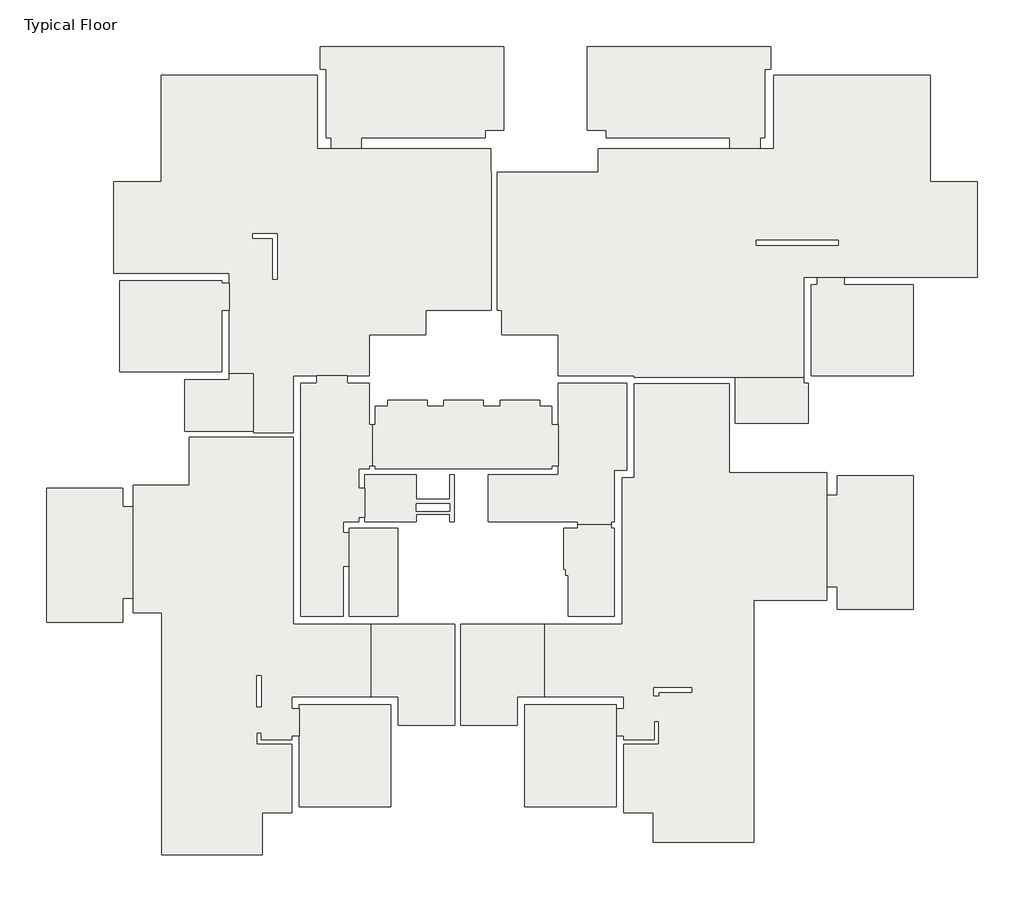
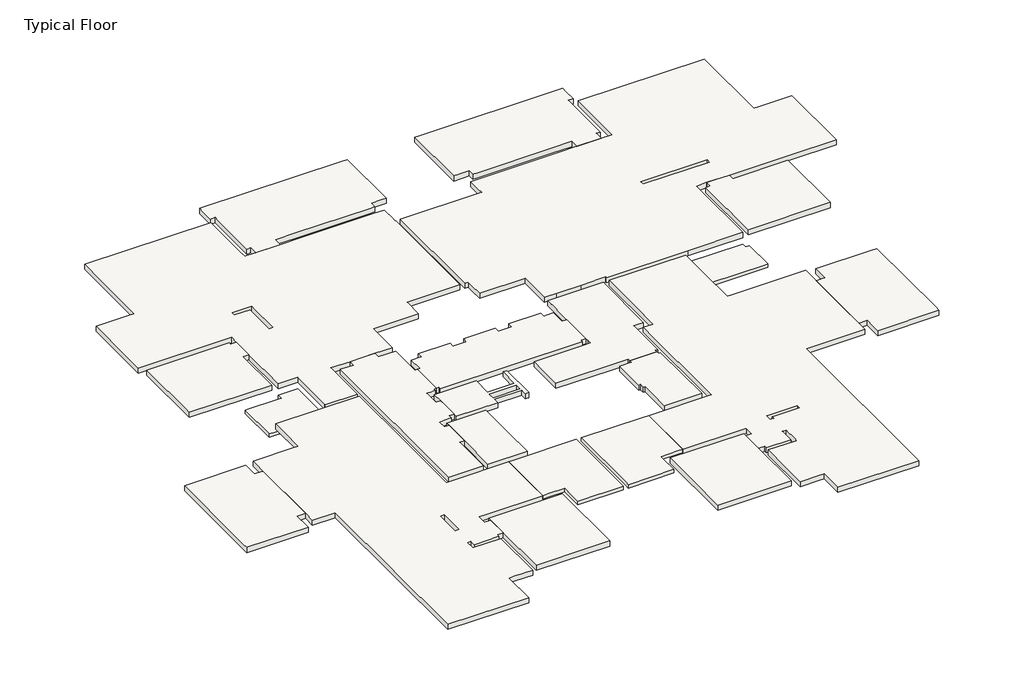
# One storey: 22 slabs.
"""IFC4 building model written with IfcOpenShell, lengths in millimetres."""

import ifcopenshell
import ifcopenshell.guid

model = None  # the IFC model being written
_history = None  # IfcOwnerHistory: only IFC2X3 demands one
_inside = {}  # id of a spatial element -> (the spatial element, [elements in it])
_under = {}  # id of a project, library or spatial element -> (it, [spatial elements below it])
_declared = {}  # id of a project -> (the project, [libraries it declares])
_typed = {}  # id of a type object -> (the type object, [elements of that type])
_made_of = {}  # id of a material, layer set ... -> (it, [elements and type objects made of it])


def new_model(schema):
    """Start an empty IFC model of exactly this schema.

    Asked for "IFC4X3", IfcOpenShell would pick the latest addendum, in which some entities
    have other attributes; the version numbers below select the first issue.
    IFC2X3 requires an IfcOwnerHistory on every rooted entity: one is made here for all.
    """
    global model, _history
    if schema == "IFC4X3":
        model = ifcopenshell.file(schema_version=(4, 3, 0, 0))
    else:
        model = ifcopenshell.file(schema=schema)
    _inside.clear()
    _under.clear()
    _declared.clear()
    _typed.clear()
    _made_of.clear()
    _history = None
    if model.schema == "IFC2X3":
        org = make("IfcOrganization", Name="unknown")
        user = make(
            "IfcPersonAndOrganization",
            ThePerson=make("IfcPerson", FamilyName="unknown"),
            TheOrganization=org,
        )
        app = make(
            "IfcApplication",
            ApplicationDeveloper=org,
            Version="unknown",
            ApplicationFullName="unknown",
            ApplicationIdentifier="unknown",
        )
        _history = make(
            "IfcOwnerHistory",
            OwningUser=user,
            OwningApplication=app,
            ChangeAction="ADDED",
            CreationDate=0,
        )
    return model


def make(cls, **values):
    """One entity of the class cls with the attributes given. An attribute that is None is left unset."""
    return model.create_entity(
        cls, **{name: value for name, value in values.items() if value is not None}
    )


def rooted(cls, **values):
    """An entity with a GlobalId (a new one), such as an element, a storey or a relation."""
    return make(cls, GlobalId=ifcopenshell.guid.new(), OwnerHistory=_history, **values)


def si_unit(unit_type, name, prefix=None):
    """IfcSIUnit, for example si_unit("LENGTHUNIT", "METRE", prefix="MILLI")."""
    return make("IfcSIUnit", UnitType=unit_type, Prefix=prefix, Name=name)


def assignment(units):
    """IfcUnitAssignment: the units of a project."""
    return None if units is None else make("IfcUnitAssignment", Units=units)


def point(xyz):
    """IfcCartesianPoint."""
    return None if xyz is None else make("IfcCartesianPoint", Coordinates=xyz)


def direction(xyz):
    """IfcDirection."""
    return None if xyz is None else make("IfcDirection", DirectionRatios=xyz)


def frame(location, z_axis=None, x_axis=None):
    """IfcAxis2Placement3D, a coordinate frame: its origin and axes. An axis left out is left unset."""
    return make(
        "IfcAxis2Placement3D",
        Location=point(location),
        Axis=direction(z_axis),
        RefDirection=direction(x_axis),
    )


def origin():
    """The frame at (0, 0, 0) with its axes left unset."""
    return frame((0.0, 0.0, 0.0))


def place(relative_to, where):
    """IfcLocalPlacement: puts the frame where relative to a parent placement (None: the world)."""
    return make(
        "IfcLocalPlacement", PlacementRelTo=relative_to, RelativePlacement=where
    )


def context(
    kind, dimensions, precision=None, world=None, true_north=None, identifier=None
):
    """IfcGeometricRepresentationContext, for example the 3D "Model" context."""
    return make(
        "IfcGeometricRepresentationContext",
        ContextIdentifier=identifier,
        ContextType=kind,
        CoordinateSpaceDimension=dimensions,
        Precision=precision,
        WorldCoordinateSystem=world,
        TrueNorth=true_north,
    )


def project(units=None, contexts=None):
    """IfcProject with its units and contexts."""
    return rooted(
        "IfcProject",
        Name="project",
        RepresentationContexts=contexts,
        UnitsInContext=assignment(units),
    )


def spatial(cls, under=None, at=None, **own):
    """A site, building, storey or space (cls), placed at a placement, below another one or the project."""
    s = rooted(cls, ObjectPlacement=at, **own)
    if under is not None:
        _under.setdefault(under.id(), (under, []))[1].append(s)
    return s


def polyline(points):
    """IfcPolyline through the points."""
    return make("IfcPolyline", Points=[point(p) for p in points])


def outline(outer, holes=None, kind="AREA"):
    """IfcArbitraryClosedProfileDef: a profile drawn as a closed curve; with holes, ...WithVoids."""
    if holes is None:
        return make("IfcArbitraryClosedProfileDef", ProfileType=kind, OuterCurve=outer)
    return make(
        "IfcArbitraryProfileDefWithVoids",
        ProfileType=kind,
        OuterCurve=outer,
        InnerCurves=holes,
    )


def extrude(swept, where, along, depth):
    """IfcExtrudedAreaSolid: the profile swept, set in the frame where, extruded along a direction by depth."""
    return make(
        "IfcExtrudedAreaSolid",
        SweptArea=swept,
        Position=where,
        ExtrudedDirection=direction(along),
        Depth=depth,
    )


def faces_of(points, faces, orient=None, outer=None):
    """IfcFace entities. A face is a list of loops; a loop is a list of indices into points, from 0.

    orient and outer hold one flag for each loop. By default every Orientation is true, the
    first loop of a face is its IfcFaceOuterBound and the others are IfcFaceBound.
    """
    made = []
    for i, loops in enumerate(faces):
        bounds = []
        for j, loop in enumerate(loops):
            is_outer = j == 0 if outer is None else outer[i][j]
            bounds.append(
                make(
                    "IfcFaceOuterBound" if is_outer else "IfcFaceBound",
                    Bound=make("IfcPolyLoop", Polygon=[points[k] for k in loop]),
                    Orientation=True if orient is None else orient[i][j],
                )
            )
        made.append(make("IfcFace", Bounds=bounds))
    return made


def faceted_brep(points, faces, orient=None, outer=None, voids=None):
    """IfcFacetedBrep: a solid bounded by flat faces; with voids (closed shells), ...WithVoids."""
    shared = [point(p) for p in points]
    hull = make("IfcClosedShell", CfsFaces=faces_of(shared, faces, orient, outer))
    if voids is None:
        return make("IfcFacetedBrep", Outer=hull)
    return make(
        "IfcFacetedBrepWithVoids",
        Outer=hull,
        Voids=[
            make(cls, CfsFaces=faces_of(shared, fs, o, b)) for cls, fs, o, b in voids
        ],
    )


def shape(context_of_items, identifier, shape_type, items):
    """IfcShapeRepresentation: the items that make up one representation, for example the "Body"."""
    return make(
        "IfcShapeRepresentation",
        ContextOfItems=context_of_items,
        RepresentationIdentifier=identifier,
        RepresentationType=shape_type,
        Items=items,
    )


def made_of(thing, what):
    """Note that an element or type object is made of a material, layer set ...; save() writes the relation."""
    if what is not None:
        _made_of.setdefault(what.id(), (what, []))[1].append(thing)
    return thing


def element(
    cls,
    number,
    at=None,
    inside=None,
    cuts=None,
    type_object=None,
    material=None,
    context=None,
    identifier="Body",
    shape_type=None,
    held_by="IfcProductDefinitionShape",
    body=None,
    shapes=None,
    **own,
):
    """One element of the class cls, such as IfcWall. Its Tag is "e" and its number.

    at: its placement. inside: the storey or other place that contains it. cuts: it is an
    opening in that element (IfcRelVoidsElement). A single representation is given by context,
    identifier, shape_type and body (its items); several are given by shapes. held_by: the class
    of the entity that holds the representations. save() writes the other relations.
    """
    e = rooted(cls, Tag="e%d" % number, ObjectPlacement=at, **own)
    if body is not None:
        shapes = [shape(context, identifier, shape_type, body)]
    if shapes is not None:
        e.Representation = make(held_by, Representations=shapes)
    if inside is not None:
        _inside.setdefault(inside.id(), (inside, []))[1].append(e)
    if cuts is not None:
        rooted(
            "IfcRelVoidsElement", RelatingBuildingElement=cuts, RelatedOpeningElement=e
        )
    if type_object is not None:
        _typed.setdefault(type_object.id(), (type_object, []))[1].append(e)
    return made_of(e, material)


def aggregate(whole, parts):
    """IfcRelAggregates: a whole, such as a stair, and the parts it consists of."""
    return rooted("IfcRelAggregates", RelatingObject=whole, RelatedObjects=parts)


def save(model, path):
    """Write the relations noted so far, then the file.

    IfcRelAggregates (storeys below a building ...), IfcRelContainedInSpatialStructure (elements
    in a storey), IfcRelDefinesByType, IfcRelAssociatesMaterial and IfcRelDeclares: one each for
    every whole, place, type object, material and project.
    """
    for whole, parts in _under.values():
        aggregate(whole, parts)
    for where, things in _inside.values():
        rooted(
            "IfcRelContainedInSpatialStructure",
            RelatedElements=things,
            RelatingStructure=where,
        )
    for kind, things in _typed.values():
        rooted("IfcRelDefinesByType", RelatedObjects=things, RelatingType=kind)
    for what, things in _made_of.values():
        rooted("IfcRelAssociatesMaterial", RelatedObjects=things, RelatingMaterial=what)
    for by, libraries in _declared.values():
        rooted("IfcRelDeclares", RelatingContext=by, RelatedDefinitions=libraries)
    model.write(path)


model = new_model("IFC4")

# Units and contexts
model_context = context("Model", 3, world=origin())
ifc_project = project(units=[si_unit("LENGTHUNIT", "METRE", prefix="MILLI")], contexts=[model_context])

# Site, building, storey
site = spatial("IfcSite", under=ifc_project)
building = spatial("IfcBuilding", under=site)
storey = spatial("IfcBuildingStorey", under=building, Name="Typical Floor", Elevation=3100.0)

# Slabs
placement = place(None, origin())
element("IfcSlab", 1, ObjectType="15", at=placement, inside=storey, context=model_context, shape_type="Brep", body=[
    faceted_brep([(26027.850174, -8804.7310591, 2300.0), (26027.850174, -9003.4933914, 2300.0), (26177.850174, -9003.4933914, 2300.0), (26177.850174, -10305.7627314, 2300.0), (23780.6220263, -10305.7627314, 2300.0), (23780.6220263, -8804.7310591, 2300.0), (26027.850174, -9003.4933914, 2450.0), (26027.850174, -8954.7310591, 2450.0), (26027.850174, -8804.7310591, 2450.0), (23780.6220263, -8804.7310591, 2450.0), (23780.6220263, -8954.7310591, 2450.0), (23780.6220263, -10305.7627314, 2450.0), (26027.850174, -10305.7627314, 2450.0), (26177.850174, -10305.7627314, 2450.0), (26177.850174, -9003.4933914, 2450.0)], [[[0, 1, 2, 3, 4, 5]], [[6, 7, 8, 9, 10, 11, 12, 13, 14]], [[1, 0, 8, 7, 6]], [[2, 1, 6, 14]], [[3, 2, 14, 13]], [[4, 3, 13, 12, 11]], [[5, 4, 11, 10, 9]], [[0, 5, 9, 8]]]),
])
element("IfcSlab", 2, ObjectType="15", at=placement, inside=storey, context=model_context, shape_type="Brep", body=[
    faceted_brep([(5696.9503171, -10574.5447275, 2300.0), (5696.9503171, -8875.9821525, 2300.0), (6907.9504595, -8875.9821525, 2300.0), (7157.9504595, -8875.9821525, 2300.0), (7157.9504595, -8673.5161743, 2300.0), (7954.0579731, -8673.5161743, 2300.0), (7954.0579731, -10574.5447275, 2300.0), (5696.9503171, -8875.9821525, 2450.0), (5696.9503171, -10574.5447275, 2450.0), (5846.9503171, -10574.5447275, 2450.0), (7804.0579731, -10574.5447275, 2450.0), (7954.0579731, -10574.5447275, 2450.0), (7954.0579731, -8873.5161743, 2450.0), (7954.0579731, -8673.5161743, 2450.0), (7157.9504595, -8673.5161743, 2450.0), (7157.9504595, -8873.5161743, 2450.0), (7157.9504595, -8875.9821525, 2450.0), (6907.9504595, -8875.9821525, 2450.0), (5846.9503171, -8875.9821525, 2450.0)], [[[0, 1, 2, 3, 4, 5, 6]], [[7, 8, 9, 10, 11, 12, 13, 14, 15, 16, 17, 18]], [[1, 0, 8, 7]], [[1, 7, 18, 17, 16, 3, 2]], [[4, 3, 16, 15, 14]], [[5, 4, 14, 13]], [[6, 5, 13, 12, 11]], [[0, 6, 11, 10, 9, 8]]]),
])
element("IfcSlab", 3, ObjectType="15", at=placement, inside=storey, context=model_context, shape_type="Brep", body=[
    faceted_brep([(11800.0437745, -19301.9218456, 2800.0), (11800.0437745, -16906.0156488, 2800.0), (12000.0437745, -16906.0156488, 2800.0), (14556.9532328, -16906.0156488, 2800.0), (14556.9532328, -20074.3060494, 2800.0), (14556.9532328, -20224.3060494, 2800.0), (12702.1320718, -20224.3060494, 2800.0), (12702.1320718, -20074.3060494, 2800.0), (12702.1320718, -19551.9218456, 2800.0), (12702.1320718, -19301.9218456, 2800.0), (12000.0437745, -19301.9218456, 2800.0), (11800.0437745, -16906.0156488, 2950.0), (11800.0437745, -19301.9218456, 2950.0), (12000.0437745, -19301.9218456, 2950.0), (12702.1320718, -19301.9218456, 2950.0), (12702.1320718, -19551.9218456, 2950.0), (12702.1320718, -20074.3060494, 2950.0), (12702.1320718, -20224.3060494, 2950.0), (14556.9532328, -20224.3060494, 2950.0), (14556.9532328, -20074.3060494, 2950.0), (14556.9532328, -16906.0156488, 2950.0), (12000.0437745, -16906.0156488, 2950.0)], [[[0, 1, 2, 3, 4, 5, 6, 7, 8, 9, 10]], [[11, 12, 13, 14, 15, 16, 17, 18, 19, 20, 21]], [[1, 0, 12, 11]], [[3, 2, 1, 11, 21, 20]], [[5, 4, 3, 20, 19, 18]], [[6, 5, 18, 17]], [[6, 17, 16, 15, 14, 9, 8, 7]], [[0, 10, 9, 14, 13, 12]]]),
])
element("IfcSlab", 4, ObjectType="15", at=placement, inside=storey, context=model_context, shape_type="Brep", body=[
    faceted_brep([(17508.6310988, -16906.0156488, 2800.0), (17508.6310988, -19301.9218456, 2800.0), (17308.6310988, -19301.9218456, 2800.0), (16611.7743938, -19301.9218456, 2800.0), (16611.7743938, -19551.9218456, 2800.0), (16611.7743938, -20074.3060494, 2800.0), (16611.7743938, -20224.3060494, 2800.0), (14756.9532328, -20224.3060494, 2800.0), (14756.9532328, -20074.3060494, 2800.0), (14756.9532328, -16906.0156488, 2800.0), (17308.6310988, -16906.0156488, 2800.0), (17508.6310988, -19301.9218456, 2950.0), (17508.6310988, -16906.0156488, 2950.0), (17308.6310988, -16906.0156488, 2950.0), (14756.9532328, -16906.0156488, 2950.0), (14756.9532328, -20074.3060494, 2950.0), (14756.9532328, -20224.3060494, 2950.0), (16611.7743938, -20224.3060494, 2950.0), (16611.7743938, -20074.3060494, 2950.0), (16611.7743938, -19551.9218456, 2950.0), (16611.7743938, -19301.9218456, 2950.0), (17308.6310988, -19301.9218456, 2950.0)], [[[0, 1, 2, 3, 4, 5, 6, 7, 8, 9, 10]], [[11, 12, 13, 14, 15, 16, 17, 18, 19, 20, 21]], [[1, 0, 12, 11]], [[3, 2, 1, 11, 21, 20]], [[3, 20, 19, 18, 17, 6, 5, 4]], [[7, 6, 17, 16]], [[9, 8, 7, 16, 15, 14]], [[0, 10, 9, 14, 13, 12]]]),
])
element("IfcSlab", 5, ObjectType="22", at=placement, inside=storey, context=model_context, shape_type="Brep", body=[
    faceted_brep([(7954.0579731, -8673.5161743, 2730.0), (7157.9504595, -8673.5161743, 2730.0), (7157.9504595, -6598.7689899, 2730.0), (7157.9504595, -5710.0703278, 2730.0), (7157.9504595, -5376.3894647, 2730.0), (6907.9504595, -5376.3894647, 2730.0), (3357.3073849, -5376.3894647, 2730.0), (3357.3073849, -2383.1380866, 2730.0), (4715.8368705, -2383.1380866, 2730.0), (4915.8368705, -2383.1380866, 2730.0), (4915.8368705, 1116.275118, 2730.0), (10045.0259753, 1116.275118, 2730.0), (10045.0259753, -935.8943434, 2730.0), (10045.0259753, -1285.8943434, 2730.0), (10497.5809154, -1285.8943434, 2730.0), (11496.1544072, -1285.8943434, 2730.0), (12338.469313, -1285.8943434, 2730.0), (15339.3043472, -1285.8943434, 2730.0), (15752.9774125, -1285.8943434, 2730.0), (15752.9774125, -1861.9790741, 2730.0), (15752.9774125, -2061.9790741, 2730.0), (15755.4299651, -2061.9790741, 2730.0), (15755.4299651, -6603.7071845, 2730.0), (13854.4950523, -6603.7071845, 2730.0), (13604.5871332, -6603.7071845, 2730.0), (13604.5871332, -7403.6947082, 2730.0), (12004.8805309, -7403.6947082, 2730.0), (11754.8805309, -7403.6947082, 2730.0), (11754.8805309, -8753.4091082, 2730.0), (11034.9623053, -8753.4091082, 2730.0), (10036.3888134, -8753.4091082, 2730.0), (9252.6267863, -8753.4091082, 2730.0), (9252.6267863, -9003.4091082, 2730.0), (9252.6267863, -10624.4557657, 2730.0), (7954.0579731, -10624.4557657, 2730.0), (7954.0579731, -10574.5447275, 2730.0), (7932.894282, -4076.5861029, 2730.0), (7932.894282, -4226.5861029, 2730.0), (8577.767247, -4226.5861029, 2730.0), (8577.767247, -5575.151797, 2730.0), (8727.767247, -5575.151797, 2730.0), (8727.767247, -4226.5861029, 2730.0), (8727.767247, -4076.5861029, 2730.0), (7157.9504595, -8673.5161743, 2950.0), (7954.0579731, -8673.5161743, 2950.0), (7954.0579731, -10574.5447275, 2950.0), (7954.0579731, -10624.4557657, 2950.0), (9252.6267863, -10624.4557657, 2950.0), (9252.6267863, -9003.4091082, 2950.0), (9252.6267863, -8753.4091082, 2950.0), (10036.3888134, -8753.4091082, 2950.0), (11034.9623053, -8753.4091082, 2950.0), (11754.8805309, -8753.4091082, 2950.0), (11754.8805309, -7403.6947082, 2950.0), (12004.8805309, -7403.6947082, 2950.0), (13604.5871332, -7403.6947082, 2950.0), (13604.5871332, -6603.7071845, 2950.0), (13854.4950523, -6603.7071845, 2950.0), (15755.4299651, -6603.7071845, 2950.0), (15755.4299651, -2061.9790741, 2950.0), (15752.9774125, -2061.9790741, 2950.0), (15752.9774125, -1861.9790741, 2950.0), (15752.9774125, -1285.8943434, 2950.0), (15339.3043472, -1285.8943434, 2950.0), (12338.469313, -1285.8943434, 2950.0), (11496.1544072, -1285.8943434, 2950.0), (10497.5809154, -1285.8943434, 2950.0), (10045.0259753, -1285.8943434, 2950.0), (10045.0259753, -935.8943434, 2950.0), (10045.0259753, 1116.275118, 2950.0), (4915.8368705, 1116.275118, 2950.0), (4915.8368705, -2383.1380866, 2950.0), (4715.8368705, -2383.1380866, 2950.0), (3357.3073849, -2383.1380866, 2950.0), (3357.3073849, -5376.3894647, 2950.0), (6907.9504595, -5376.3894647, 2950.0), (7157.9504595, -5376.3894647, 2950.0), (7157.9504595, -5710.0703278, 2950.0), (7157.9504595, -6598.7689899, 2950.0), (7932.894282, -4226.5861029, 2950.0), (7932.894282, -4076.5861029, 2950.0), (8727.767247, -4076.5861029, 2950.0), (8727.767247, -4226.5861029, 2950.0), (8727.767247, -5575.151797, 2950.0), (8577.767247, -5575.151797, 2950.0), (8577.767247, -4226.5861029, 2950.0), (7954.0579731, -8673.5161743, 2900.0), (7157.9504595, -8673.5161743, 2900.0)], [[[0, 1, 2, 3, 4, 5, 6, 7, 8, 9, 10, 11, 12, 13, 14, 15, 16, 17, 18, 19, 20, 21, 22, 23, 24, 25, 26, 27, 28, 29, 30, 31, 32, 33, 34, 35], [36, 37, 38, 39, 40, 41, 42]], [[43, 44, 45, 46, 47, 48, 49, 50, 51, 52, 53, 54, 55, 56, 57, 58, 59, 60, 61, 62, 63, 64, 65, 66, 67, 68, 69, 70, 71, 72, 73, 74, 75, 76, 77, 78], [79, 80, 81, 82, 83, 84, 85]], [[1, 0, 86, 44, 43, 87]], [[1, 87, 43, 78, 77, 76, 4, 3, 2]], [[4, 76, 75, 74, 6, 5]], [[7, 6, 74, 73]], [[7, 73, 72, 71, 9, 8]], [[10, 9, 71, 70]], [[11, 10, 70, 69]], [[11, 69, 68, 67, 13, 12]], [[13, 67, 66, 65, 64, 63, 62, 18, 17, 16, 15, 14]], [[18, 62, 61, 60, 20, 19]], [[21, 20, 60, 59]], [[22, 21, 59, 58]], [[22, 58, 57, 56, 24, 23]], [[25, 24, 56, 55]], [[25, 55, 54, 53, 27, 26]], [[28, 27, 53, 52]], [[28, 52, 51, 50, 49, 31, 30, 29]], [[31, 49, 48, 47, 33, 32]], [[34, 33, 47, 46]], [[35, 34, 46, 45]], [[0, 35, 45, 44, 86]], [[37, 36, 80, 79]], [[38, 37, 79, 85]], [[39, 38, 85, 84]], [[40, 39, 84, 83]], [[40, 83, 82, 81, 42, 41]], [[36, 42, 81, 80]]]),
])
element("IfcSlab", 6, ObjectType="22", at=placement, inside=storey, context=model_context, shape_type="Brep", body=[
    faceted_brep([(25049.2058247, 1116.275118, 2730.0), (30178.3996082, 1116.275118, 2730.0), (30178.3996082, -2383.1380866, 2730.0), (30378.3996082, -2383.1380866, 2730.0), (31735.6945451, -2383.1380866, 2730.0), (31735.6945451, -5506.3666818, 2730.0), (29827.2587, -5506.3666818, 2730.0), (27367.2587, -5506.3666818, 2730.0), (26467.7022208, -5506.3666818, 2730.0), (26027.850174, -5506.3666818, 2730.0), (26027.850174, -5756.3666818, 2730.0), (26027.850174, -8804.7310591, 2730.0), (23780.6220263, -8804.7310591, 2730.0), (20461.0939579, -8804.7310591, 2730.0), (20461.0939579, -8753.4091082, 2730.0), (20211.0939579, -8753.4091082, 2730.0), (19458.8168201, -8753.4091082, 2730.0), (18458.8324156, -8753.4091082, 2730.0), (17955.1365674, -8753.4091082, 2730.0), (17955.1365674, -7653.6026273, 2730.0), (17955.1365674, -7403.6026273, 2730.0), (16105.4299651, -7403.6026273, 2730.0), (16105.4299651, -6853.7071845, 2730.0), (16105.4299651, -6603.7071845, 2730.0), (15955.4299651, -6603.7071845, 2730.0), (15955.4299651, -2061.9790741, 2730.0), (19272.5763384, -2061.9790741, 2730.0), (19272.5763384, -1861.9790741, 2730.0), (19272.5763384, -1287.0352516, 2730.0), (19754.9321315, -1287.0352516, 2730.0), (22755.7671656, -1287.0352516, 2730.0), (23598.2584356, -1287.0352516, 2730.0), (24600.5355733, -1287.0352516, 2730.0), (25049.2058247, -1287.0352516, 2730.0), (25049.2058247, -937.0352516, 2730.0), (27166.4567553, -4305.3303309, 2730.0), (24469.3206885, -4305.3303309, 2730.0), (24469.3206885, -4455.3303309, 2730.0), (27166.4567553, -4455.3303309, 2730.0), (30178.3996082, 1116.275118, 2950.0), (25049.2058247, 1116.275118, 2950.0), (25049.2058247, -937.0352516, 2950.0), (25049.2058247, -1287.0352516, 2950.0), (24600.5355733, -1287.0352516, 2950.0), (23598.2584356, -1287.0352516, 2950.0), (22755.7671656, -1287.0352516, 2950.0), (19754.9321315, -1287.0352516, 2950.0), (19272.5763384, -1287.0352516, 2950.0), (19272.5763384, -1861.9790741, 2950.0), (19272.5763384, -2061.9790741, 2950.0), (15955.4299651, -2061.9790741, 2950.0), (15955.4299651, -6603.7071845, 2950.0), (16105.4299651, -6603.7071845, 2950.0), (16105.4299651, -6853.7071845, 2950.0), (16105.4299651, -7403.6026273, 2950.0), (17955.1365674, -7403.6026273, 2950.0), (17955.1365674, -7653.6026273, 2950.0), (17955.1365674, -8753.4091082, 2950.0), (18458.8324156, -8753.4091082, 2950.0), (19458.8168201, -8753.4091082, 2950.0), (20211.0939579, -8753.4091082, 2950.0), (20461.0939579, -8753.4091082, 2950.0), (20461.0939579, -8804.7310591, 2950.0), (23780.6220263, -8804.7310591, 2950.0), (26027.850174, -8804.7310591, 2950.0), (26027.850174, -5756.3666818, 2950.0), (26027.850174, -5506.3666818, 2950.0), (26467.7022208, -5506.3666818, 2950.0), (27367.2587, -5506.3666818, 2950.0), (29827.2587, -5506.3666818, 2950.0), (31735.6945451, -5506.3666818, 2950.0), (31735.6945451, -2383.1380866, 2950.0), (30378.3996082, -2383.1380866, 2950.0), (30178.3996082, -2383.1380866, 2950.0), (24469.3206885, -4305.3303309, 2950.0), (27166.4567553, -4305.3303309, 2950.0), (27166.4567553, -4455.3303309, 2950.0), (24469.3206885, -4455.3303309, 2950.0), (26027.850174, -8804.7310591, 2900.0)], [[[0, 1, 2, 3, 4, 5, 6, 7, 8, 9, 10, 11, 12, 13, 14, 15, 16, 17, 18, 19, 20, 21, 22, 23, 24, 25, 26, 27, 28, 29, 30, 31, 32, 33, 34], [35, 36, 37, 38]], [[39, 40, 41, 42, 43, 44, 45, 46, 47, 48, 49, 50, 51, 52, 53, 54, 55, 56, 57, 58, 59, 60, 61, 62, 63, 64, 65, 66, 67, 68, 69, 70, 71, 72, 73], [74, 75, 76, 77]], [[47, 28, 27, 26, 49, 48]], [[28, 47, 46, 45, 44, 31, 30, 29]], [[31, 44, 43, 42, 33, 32]], [[33, 42, 41, 40, 0, 34]], [[1, 0, 40, 39]], [[2, 1, 39, 73]], [[2, 73, 72, 71, 4, 3]], [[5, 4, 71, 70]], [[5, 70, 69, 68, 7, 6]], [[8, 7, 68, 67]], [[9, 8, 67, 66]], [[9, 66, 65, 64, 78, 11, 10]], [[13, 12, 63, 62]], [[14, 13, 62, 61]], [[14, 61, 60, 59, 16, 15]], [[17, 16, 59, 58]], [[18, 17, 58, 57]], [[18, 57, 56, 55, 20, 19]], [[21, 20, 55, 54]], [[21, 54, 53, 52, 23, 22]], [[24, 23, 52, 51]], [[25, 24, 51, 50]], [[26, 25, 50, 49]], [[12, 11, 78, 64, 63]], [[36, 35, 75, 74]], [[37, 36, 74, 77]], [[38, 37, 77, 76]], [[35, 38, 76, 75]]]),
])
element("IfcSlab", 7, ObjectType="22", at=placement, inside=storey, context=model_context, shape_type="Brep", body=[
    faceted_brep([(19861.1907174, -19551.9218456, 2730.0), (19861.1907174, -19695.7428642, 2730.0), (19861.1907174, -20584.2651623, 2730.0), (19861.1907174, -22902.7444034, 2730.0), (16861.7743938, -22902.7444034, 2730.0), (16861.7743938, -19551.9218456, 2730.0), (19861.1907174, -19551.9218456, 2950.0), (16861.7743938, -19551.9218456, 2950.0), (16861.7743938, -22902.7444034, 2950.0), (19861.1907174, -22902.7444034, 2950.0), (19861.1907174, -20584.2651623, 2950.0), (19861.1907174, -19695.7428642, 2950.0)], [[[0, 1, 2, 3, 4, 5]], [[6, 7, 8, 9, 10, 11]], [[3, 2, 1, 0, 6, 11, 10, 9]], [[4, 3, 9, 8]], [[5, 4, 8, 7]], [[0, 5, 7, 6]]]),
])
element("IfcSlab", 8, ObjectType="22", at=placement, inside=storey, context=model_context, shape_type="Brep", body=[
    faceted_brep([(9452.7157481, -19551.9218456, 2730.0), (12452.1320718, -19551.9218456, 2730.0), (12452.1320718, -22902.7444034, 2730.0), (9452.7157481, -22902.7444034, 2730.0), (9452.7157481, -20584.2651623, 2730.0), (9452.7157481, -19695.7428642, 2730.0), (9452.7157481, -19551.9218456, 2950.0), (9452.7157481, -19695.7428642, 2950.0), (9452.7157481, -20584.2651623, 2950.0), (9452.7157481, -22902.7444034, 2950.0), (12452.1320718, -22902.7444034, 2950.0), (12452.1320718, -19551.9218456, 2950.0)], [[[0, 1, 2, 3, 4, 5]], [[6, 7, 8, 9, 10, 11]], [[1, 0, 6, 11]], [[2, 1, 11, 10]], [[3, 2, 10, 9]], [[0, 5, 4, 3, 9, 8, 7, 6]]]),
])
element("IfcSlab", 9, ObjectType="22", at=placement, inside=storey, context=model_context, shape_type="SweptSolid", body=[
    extrude(outline(polyline([(13654.4981714, -9553.3966318), (13654.4981714, -9753.3966318), (14205.8123246, -9753.3966318), (14205.8123246, -9553.3966318), (15504.3811378, -9553.3966318), (15504.3811378, -9753.3966318), (16055.5189269, -9753.3966318), (16055.5189269, -9553.3966318), (17354.0877401, -9553.3966318), (17354.0877401, -9753.3935127), (17755.1365674, -9753.3935127), (17755.1365674, -10353.2077914), (17955.1365674, -10353.2077914), (17955.1365674, -11704.3331041), (17755.1365674, -11704.3331041), (17755.1365674, -11804.3284255), (11954.8805309, -11804.3284255), (11954.8805309, -11704.3331041), (11854.8805309, -11704.3331041), (11854.8805309, -10353.2077914), (11954.8805309, -10353.2077914), (11954.8805309, -9753.3966318), (12355.9293582, -9753.3966318), (12355.9293582, -9553.3966318), (13654.4981714, -9553.3966318)])), frame((0.0, 0.0, 2730.0), z_axis=(0.0, 0.0, 1.0), x_axis=(1.0, 0.0, 0.0)), (0.0, 0.0, 1.0), 220.0),
])
element("IfcSlab", 10, ObjectType="22", at=placement, inside=storey, context=model_context, shape_type="Brep", body=[
    faceted_brep([(20211.0939579, -9003.4091082, 2730.0), (20211.0939579, -11856.7116801, 2730.0), (20059.9577283, -11856.7116801, 2730.0), (19809.9577283, -11856.7116801, 2730.0), (19808.6310988, -11856.7116801, 2730.0), (19808.6310988, -13252.8098364, 2730.0), (19808.6310988, -13552.8020387, 2730.0), (19712.4283852, -13552.8020387, 2730.0), (19712.4283852, -13652.8020387, 2730.0), (18611.3873556, -13652.8020387, 2730.0), (18611.3873556, -13552.8020387, 2730.0), (15663.7943424, -13552.8020387, 2730.0), (15663.7943424, -12004.3284255, 2730.0), (17755.1365674, -12004.3284255, 2730.0), (17955.1365674, -12004.3284255, 2730.0), (17955.1365674, -11856.7116801, 2730.0), (17955.1365674, -11704.3331041, 2730.0), (17955.1365674, -10353.2077914, 2730.0), (17955.1365674, -9753.3935127, 2730.0), (17955.1365674, -9553.3935127, 2730.0), (17955.1365674, -9003.4091082, 2730.0), (20211.0939579, -11856.7116801, 2950.0), (20211.0939579, -9003.4091082, 2950.0), (17955.1365674, -9003.4091082, 2950.0), (17955.1365674, -9553.3935127, 2950.0), (17955.1365674, -9753.3935127, 2950.0), (17955.1365674, -10353.2077914, 2950.0), (17955.1365674, -11704.3331041, 2950.0), (17955.1365674, -11856.7116801, 2950.0), (17955.1365674, -12004.3284255, 2950.0), (17755.1365674, -12004.3284255, 2950.0), (15663.7943424, -12004.3284255, 2950.0), (15663.7943424, -13552.8020387, 2950.0), (18611.3873556, -13552.8020387, 2950.0), (18611.3873556, -13652.8020387, 2950.0), (19712.4283852, -13652.8020387, 2950.0), (19712.4283852, -13552.8020387, 2950.0), (19808.6310988, -13552.8020387, 2950.0), (19808.6310988, -13252.8098364, 2950.0), (19808.6310988, -11856.7116801, 2950.0), (19809.9577283, -11856.7116801, 2950.0), (20059.9577283, -11856.7116801, 2950.0)], [[[0, 1, 2, 3, 4, 5, 6, 7, 8, 9, 10, 11, 12, 13, 14, 15, 16, 17, 18, 19, 20]], [[21, 22, 23, 24, 25, 26, 27, 28, 29, 30, 31, 32, 33, 34, 35, 36, 37, 38, 39, 40, 41]], [[1, 0, 22, 21]], [[1, 21, 41, 40, 39, 4, 3, 2]], [[5, 4, 39, 38]], [[6, 5, 38, 37]], [[7, 6, 37, 36]], [[8, 7, 36, 35]], [[9, 8, 35, 34]], [[10, 9, 34, 33]], [[11, 10, 33, 32]], [[12, 11, 32, 31]], [[12, 31, 30, 29, 14, 13]], [[15, 14, 29, 28]], [[15, 28, 27, 26, 25, 24, 23, 20, 19, 18, 17, 16]], [[0, 20, 23, 22]]]),
])
element("IfcSlab", 11, ObjectType="22", at=placement, inside=storey, context=model_context, shape_type="SweptSolid", body=[
    extrude(outline(polyline([(13299.6536172, -12004.3284255), (13299.6536172, -12804.3284255), (14404.6536172, -12804.3284255), (14404.6536172, -12004.3284255), (14544.6536172, -12004.3284255), (14544.6536172, -13552.8020387), (14404.6536172, -13552.8020387), (14404.6536172, -13302.8020387), (13294.6536172, -13302.8020387), (13294.6536172, -13552.8020387), (11603.5632586, -13552.8020387), (11603.5632586, -13405.3647765), (11603.5632586, -12452.9986769), (11603.5632586, -12004.3284255), (13299.6536172, -12004.3284255)]), holes=[polyline([(14399.4600982, -12952.8145151), (13299.6536172, -12952.8145151), (13299.6536172, -13202.8987982), (14399.4600982, -13202.8987982), (14399.4600982, -12952.8145151)])]), frame((0.0, 0.0, 2730.0), z_axis=(0.0, 0.0, 1.0), x_axis=(1.0, 0.0, 0.0)), (0.0, 0.0, 1.0), 220.0),
])
element("IfcSlab", 12, ObjectType="22", at=placement, inside=storey, context=model_context, shape_type="SweptSolid", body=[
    extrude(outline(polyline([(18141.3770491, -15102.5164387), (18141.3770491, -13752.8020387), (18611.3873556, -13752.8020387), (18611.3873556, -13652.8020387), (19712.4283852, -13652.8020387), (19712.4283852, -13752.8020387), (19808.6310988, -13752.8020387), (19808.6310988, -16655.7368174), (18287.5813222, -16655.7368174), (18287.5813222, -15306.2169656), (18213.8626911, -15306.2169656), (18213.8626911, -15106.2169656), (18141.3770491, -15106.2169656), (18141.3770491, -15102.5164387)])), frame((0.0, 0.0, 2730.0), z_axis=(0.0, 0.0, 1.0), x_axis=(1.0, 0.0, 0.0)), (0.0, 0.0, 1.0), 220.0),
])
element("IfcSlab", 13, ObjectType="22", at=placement, inside=storey, context=model_context, shape_type="SweptSolid", body=[
    extrude(outline(polyline([(12694.7247799, -15306.2169656), (12694.7247799, -16656.0156488), (11100.0437745, -16656.0156488), (11100.0437745, -15005.1634597), (11100.0437745, -13905.1806146), (11100.0437745, -13752.8020387), (12694.7247799, -13752.8020387), (12694.7247799, -15306.2169656)])), frame((0.0, 0.0, 2730.0), z_axis=(0.0, 0.0, 1.0), x_axis=(1.0, 0.0, 0.0)), (0.0, 0.0, 1.0), 220.0),
])
element("IfcSlab", 14, ObjectType="22", at=placement, inside=storey, context=model_context, shape_type="Brep", body=[
    faceted_brep([(10036.3888134, -9003.4091082, 2730.0), (10036.3888134, -8753.4091082, 2730.0), (11034.9623053, -8753.4091082, 2730.0), (11034.9623053, -9003.4091082, 2730.0), (11754.8805309, -9003.4091082, 2730.0), (11754.8805309, -9553.3966318, 2730.0), (11754.8805309, -9753.3966318, 2730.0), (11754.8805309, -10353.2077914, 2730.0), (11854.8805309, -10353.2077914, 2730.0), (11854.8805309, -11704.3331041, 2730.0), (11754.8805309, -11704.3331041, 2730.0), (11754.8805309, -11804.3284255, 2730.0), (11603.5632586, -11804.3284255, 2730.0), (11403.5632586, -11804.3284255, 2730.0), (11403.5632586, -12452.9986769, 2730.0), (11603.5632586, -12452.9986769, 2730.0), (11603.5632586, -13405.3647765, 2730.0), (11403.5632586, -13405.3647765, 2730.0), (11403.5632586, -13552.8020387, 2730.0), (11100.0437745, -13552.8020387, 2730.0), (10900.0437745, -13552.8020387, 2730.0), (10900.0437745, -13905.1806146, 2730.0), (11100.0437745, -13905.1806146, 2730.0), (11100.0437745, -15005.1634597, 2730.0), (10900.0437745, -15005.1634597, 2730.0), (10900.0437745, -16656.0156488, 2730.0), (9502.6267863, -16656.0156488, 2730.0), (9502.6267863, -9003.4091082, 2730.0), (10036.3888134, -8753.4091082, 2950.0), (10036.3888134, -9003.4091082, 2950.0), (9502.6267863, -9003.4091082, 2950.0), (9502.6267863, -16656.0156488, 2950.0), (10900.0437745, -16656.0156488, 2950.0), (10900.0437745, -15005.1634597, 2950.0), (11100.0437745, -15005.1634597, 2950.0), (11100.0437745, -13905.1806146, 2950.0), (10900.0437745, -13905.1806146, 2950.0), (10900.0437745, -13552.8020387, 2950.0), (11100.0437745, -13552.8020387, 2950.0), (11403.5632586, -13552.8020387, 2950.0), (11403.5632586, -13405.3647765, 2950.0), (11603.5632586, -13405.3647765, 2950.0), (11603.5632586, -12452.9986769, 2950.0), (11403.5632586, -12452.9986769, 2950.0), (11403.5632586, -11804.3284255, 2950.0), (11603.5632586, -11804.3284255, 2950.0), (11754.8805309, -11804.3284255, 2950.0), (11754.8805309, -11704.3331041, 2950.0), (11854.8805309, -11704.3331041, 2950.0), (11854.8805309, -10353.2077914, 2950.0), (11754.8805309, -10353.2077914, 2950.0), (11754.8805309, -9753.3966318, 2950.0), (11754.8805309, -9553.3966318, 2950.0), (11754.8805309, -9003.4091082, 2950.0), (11034.9623053, -9003.4091082, 2950.0), (11034.9623053, -8753.4091082, 2950.0)], [[[0, 1, 2, 3, 4, 5, 6, 7, 8, 9, 10, 11, 12, 13, 14, 15, 16, 17, 18, 19, 20, 21, 22, 23, 24, 25, 26, 27]], [[28, 29, 30, 31, 32, 33, 34, 35, 36, 37, 38, 39, 40, 41, 42, 43, 44, 45, 46, 47, 48, 49, 50, 51, 52, 53, 54, 55]], [[1, 0, 29, 28]], [[2, 1, 28, 55]], [[3, 2, 55, 54]], [[4, 3, 54, 53]], [[4, 53, 52, 51, 50, 7, 6, 5]], [[8, 7, 50, 49]], [[9, 8, 49, 48]], [[10, 9, 48, 47]], [[11, 10, 47, 46]], [[11, 46, 45, 44, 13, 12]], [[14, 13, 44, 43]], [[15, 14, 43, 42]], [[16, 15, 42, 41]], [[17, 16, 41, 40]], [[18, 17, 40, 39]], [[18, 39, 38, 37, 20, 19]], [[21, 20, 37, 36]], [[22, 21, 36, 35]], [[23, 22, 35, 34]], [[24, 23, 34, 33]], [[25, 24, 33, 32]], [[26, 25, 32, 31]], [[27, 26, 31, 30]], [[0, 27, 30, 29]]]),
])
element("IfcSlab", 15, ObjectType="22", at=placement, inside=storey, context=model_context, shape_type="Brep", body=[
    faceted_brep([(9202.7157481, -19301.9218456, 2730.0), (9202.7157481, -19695.7428642, 2730.0), (9452.7157481, -19695.7428642, 2730.0), (9452.7157481, -20584.2651623, 2730.0), (9202.7157481, -20584.2651623, 2730.0), (9202.7157481, -20705.5131366, 2730.0), (8200.3527676, -20705.5131366, 2730.0), (8200.3527676, -20474.3903326, 2730.0), (8050.3527676, -20474.3903326, 2730.0), (8050.3527676, -20705.5131366, 2730.0), (8050.3527676, -20855.5131366, 2730.0), (9202.7157481, -20855.5131366, 2730.0), (9202.7157481, -23102.7444034, 2730.0), (8431.4755716, -23102.7444034, 2730.0), (8231.4755716, -23102.7444034, 2730.0), (8231.4755716, -24493.724882, 2730.0), (4932.0592479, -24493.724882, 2730.0), (4932.0592479, -16842.3482114, 2730.0), (4932.0592479, -16542.3482114, 2730.0), (4004.7368494, -16542.3482114, 2730.0), (4004.7368494, -16059.997097, 2730.0), (4004.7368494, -13054.0475042, 2730.0), (4004.7368494, -12353.0033555, 2730.0), (5645.6252471, -12353.0033555, 2730.0), (5845.6252471, -12353.0033555, 2730.0), (5845.6252471, -10774.5447275, 2730.0), (9252.6267863, -10774.5447275, 2730.0), (9252.6267863, -13892.8351282, 2730.0), (9252.6267863, -14895.1122659, 2730.0), (9252.6267863, -16906.0156488, 2730.0), (9502.7110695, -16906.0156488, 2730.0), (11800.0437745, -16906.0156488, 2730.0), (11800.0437745, -19301.9218456, 2730.0), (9452.7157481, -19301.9218456, 2730.0), (8200.3527676, -18603.3436751, 2730.0), (8050.3527676, -18603.3436751, 2730.0), (8050.3527676, -19623.2572222, 2730.0), (8200.3527676, -19623.2572222, 2730.0), (9202.7157481, -19695.7428642, 2950.0), (9202.7157481, -19301.9218456, 2950.0), (9452.7157481, -19301.9218456, 2950.0), (11800.0437745, -19301.9218456, 2950.0), (11800.0437745, -16906.0156488, 2950.0), (9502.7110695, -16906.0156488, 2950.0), (9252.6267863, -16906.0156488, 2950.0), (9252.6267863, -14895.1122659, 2950.0), (9252.6267863, -13892.8351282, 2950.0), (9252.6267863, -10774.5447275, 2950.0), (5845.6252471, -10774.5447275, 2950.0), (5845.6252471, -12353.0033555, 2950.0), (5645.6252471, -12353.0033555, 2950.0), (4004.7368494, -12353.0033555, 2950.0), (4004.7368494, -13054.0475042, 2950.0), (4004.7368494, -16059.997097, 2950.0), (4004.7368494, -16542.3482114, 2950.0), (4932.0592479, -16542.3482114, 2950.0), (4932.0592479, -16842.3482114, 2950.0), (4932.0592479, -24493.724882, 2950.0), (8231.4755716, -24493.724882, 2950.0), (8231.4755716, -23102.7444034, 2950.0), (8431.4755716, -23102.7444034, 2950.0), (9202.7157481, -23102.7444034, 2950.0), (9202.7157481, -20855.5131366, 2950.0), (8050.3527676, -20855.5131366, 2950.0), (8050.3527676, -20705.5131366, 2950.0), (8050.3527676, -20474.3903326, 2950.0), (8200.3527676, -20474.3903326, 2950.0), (8200.3527676, -20705.5131366, 2950.0), (9202.7157481, -20705.5131366, 2950.0), (9202.7157481, -20584.2651623, 2950.0), (9452.7157481, -20584.2651623, 2950.0), (9452.7157481, -19695.7428642, 2950.0), (8050.3527676, -18603.3436751, 2950.0), (8200.3527676, -18603.3436751, 2950.0), (8200.3527676, -19623.2572222, 2950.0), (8050.3527676, -19623.2572222, 2950.0), (11800.0437745, -19301.9218456, 2750.0), (11800.0437745, -19301.9218456, 2800.0), (11800.0437745, -16906.0156488, 2800.0), (11800.0437745, -16906.0156488, 2750.0)], [[[0, 1, 2, 3, 4, 5, 6, 7, 8, 9, 10, 11, 12, 13, 14, 15, 16, 17, 18, 19, 20, 21, 22, 23, 24, 25, 26, 27, 28, 29, 30, 31, 32, 33], [34, 35, 36, 37]], [[38, 39, 40, 41, 42, 43, 44, 45, 46, 47, 48, 49, 50, 51, 52, 53, 54, 55, 56, 57, 58, 59, 60, 61, 62, 63, 64, 65, 66, 67, 68, 69, 70, 71], [72, 73, 74, 75]], [[39, 0, 33, 32, 76, 77, 41, 40]], [[1, 0, 39, 38]], [[2, 1, 38, 71]], [[3, 2, 71, 70]], [[4, 3, 70, 69]], [[5, 4, 69, 68]], [[6, 5, 68, 67]], [[7, 6, 67, 66]], [[8, 7, 66, 65]], [[8, 65, 64, 63, 10, 9]], [[11, 10, 63, 62]], [[12, 11, 62, 61]], [[12, 61, 60, 59, 14, 13]], [[15, 14, 59, 58]], [[16, 15, 58, 57]], [[16, 57, 56, 55, 18, 17]], [[19, 18, 55, 54]], [[22, 21, 20, 19, 54, 53, 52, 51]], [[22, 51, 50, 49, 24, 23]], [[25, 24, 49, 48]], [[26, 25, 48, 47]], [[26, 47, 46, 45, 44, 29, 28, 27]], [[29, 44, 43, 42, 78, 79, 31, 30]], [[32, 31, 79, 78, 42, 41, 77, 76]], [[35, 34, 73, 72]], [[36, 35, 72, 75]], [[37, 36, 75, 74]], [[34, 37, 74, 73]]]),
])
element("IfcSlab", 16, ObjectType="22", at=placement, inside=storey, context=model_context, shape_type="Brep", body=[
    faceted_brep([(17508.6310988, -19301.9218456, 2730.0), (17508.6310988, -16906.0156488, 2730.0), (20058.6310988, -16906.0156488, 2730.0), (20059.9577283, -16906.0156488, 2730.0), (20059.9577283, -12254.2363446, 2730.0), (20059.9577283, -12106.7116801, 2730.0), (20461.0939579, -12106.7116801, 2730.0), (20461.0939579, -11856.7116801, 2730.0), (20461.0939579, -9004.7310591, 2730.0), (23580.6220263, -9004.7310591, 2730.0), (23580.6220263, -10650.7340155, 2730.0), (23580.6220263, -11585.6400699, 2730.0), (23580.6220263, -11933.0804512, 2730.0), (23780.6220263, -11933.0804512, 2730.0), (26777.656655, -11933.0804512, 2730.0), (26777.656655, -12677.8628948, 2730.0), (26777.656655, -15678.697929, 2730.0), (26777.656655, -16118.7263398, 2730.0), (24582.430894, -16118.7263398, 2730.0), (24382.430894, -16118.7263398, 2730.0), (24382.430894, -24077.7444034, 2730.0), (21082.430894, -24077.7444034, 2730.0), (21082.430894, -23102.7444034, 2730.0), (20882.430894, -23102.7444034, 2730.0), (20111.1907174, -23102.7444034, 2730.0), (20111.1907174, -20855.5131366, 2730.0), (21263.5536979, -20855.5131366, 2730.0), (21263.5536979, -20705.5131366, 2730.0), (21263.5536979, -20105.5131366, 2730.0), (21113.5536979, -20105.5131366, 2730.0), (21113.5536979, -20705.5131366, 2730.0), (20111.1907174, -20705.5131366, 2730.0), (20111.1907174, -20584.2651623, 2730.0), (19861.1907174, -20584.2651623, 2730.0), (19861.1907174, -19695.7428642, 2730.0), (20111.1907174, -19695.7428642, 2730.0), (20111.1907174, -19301.9218456, 2730.0), (19861.1907174, -19301.9218456, 2730.0), (21108.5265415, -19255.7144534, 2730.0), (21258.5265415, -19255.7144534, 2730.0), (21258.5265415, -19155.8065343, 2730.0), (22357.1843165, -19155.8065343, 2730.0), (22357.1843165, -19005.8065343, 2730.0), (21258.5265415, -19005.8065343, 2730.0), (21108.5265415, -19005.8065343, 2730.0), (17508.6310988, -16906.0156488, 2950.0), (17508.6310988, -19301.9218456, 2950.0), (19861.1907174, -19301.9218456, 2950.0), (20111.1907174, -19301.9218456, 2950.0), (20111.1907174, -19695.7428642, 2950.0), (19861.1907174, -19695.7428642, 2950.0), (19861.1907174, -20584.2651623, 2950.0), (20111.1907174, -20584.2651623, 2950.0), (20111.1907174, -20705.5131366, 2950.0), (21113.5536979, -20705.5131366, 2950.0), (21113.5536979, -20105.5131366, 2950.0), (21263.5536979, -20105.5131366, 2950.0), (21263.5536979, -20705.5131366, 2950.0), (21263.5536979, -20855.5131366, 2950.0), (20111.1907174, -20855.5131366, 2950.0), (20111.1907174, -23102.7444034, 2950.0), (20882.430894, -23102.7444034, 2950.0), (21082.430894, -23102.7444034, 2950.0), (21082.430894, -24077.7444034, 2950.0), (24382.430894, -24077.7444034, 2950.0), (24382.430894, -16118.7263398, 2950.0), (24582.430894, -16118.7263398, 2950.0), (26777.656655, -16118.7263398, 2950.0), (26777.656655, -15678.697929, 2950.0), (26777.656655, -12677.8628948, 2950.0), (26777.656655, -11933.0804512, 2950.0), (23780.6220263, -11933.0804512, 2950.0), (23580.6220263, -11933.0804512, 2950.0), (23580.6220263, -11585.6400699, 2950.0), (23580.6220263, -10650.7340155, 2950.0), (23580.6220263, -9004.7310591, 2950.0), (20461.0939579, -9004.7310591, 2950.0), (20461.0939579, -11856.7116801, 2950.0), (20461.0939579, -12106.7116801, 2950.0), (20059.9577283, -12106.7116801, 2950.0), (20059.9577283, -12254.2363446, 2950.0), (20059.9577283, -16906.0156488, 2950.0), (20058.6310988, -16906.0156488, 2950.0), (21258.5265415, -19255.7144534, 2950.0), (21108.5265415, -19255.7144534, 2950.0), (21108.5265415, -19005.8065343, 2950.0), (21258.5265415, -19005.8065343, 2950.0), (22357.1843165, -19005.8065343, 2950.0), (22357.1843165, -19155.8065343, 2950.0), (21258.5265415, -19155.8065343, 2950.0), (17508.6310988, -19301.9218456, 2750.0), (17508.6310988, -19301.9218456, 2800.0), (17508.6310988, -16906.0156488, 2800.0), (17508.6310988, -16906.0156488, 2750.0)], [[[0, 1, 2, 3, 4, 5, 6, 7, 8, 9, 10, 11, 12, 13, 14, 15, 16, 17, 18, 19, 20, 21, 22, 23, 24, 25, 26, 27, 28, 29, 30, 31, 32, 33, 34, 35, 36, 37], [38, 39, 40, 41, 42, 43, 44]], [[45, 46, 47, 48, 49, 50, 51, 52, 53, 54, 55, 56, 57, 58, 59, 60, 61, 62, 63, 64, 65, 66, 67, 68, 69, 70, 71, 72, 73, 74, 75, 76, 77, 78, 79, 80, 81, 82], [83, 84, 85, 86, 87, 88, 89]], [[1, 0, 90, 91, 46, 45, 92, 93]], [[1, 93, 92, 45, 82, 81, 3, 2]], [[3, 81, 80, 79, 5, 4]], [[6, 5, 79, 78]], [[6, 78, 77, 76, 8, 7]], [[9, 8, 76, 75]], [[9, 75, 74, 73, 72, 12, 11, 10]], [[12, 72, 71, 70, 14, 13]], [[17, 16, 15, 14, 70, 69, 68, 67]], [[17, 67, 66, 65, 19, 18]], [[20, 19, 65, 64]], [[21, 20, 64, 63]], [[22, 21, 63, 62]], [[22, 62, 61, 60, 24, 23]], [[25, 24, 60, 59]], [[26, 25, 59, 58]], [[26, 58, 57, 56, 28, 27]], [[29, 28, 56, 55]], [[30, 29, 55, 54]], [[31, 30, 54, 53]], [[32, 31, 53, 52]], [[33, 32, 52, 51]], [[34, 33, 51, 50]], [[35, 34, 50, 49]], [[36, 35, 49, 48]], [[36, 48, 47, 46, 91, 90, 0, 37]], [[39, 38, 84, 83]], [[40, 39, 83, 89]], [[41, 40, 89, 88]], [[42, 41, 88, 87]], [[42, 87, 86, 85, 44, 43]], [[38, 44, 85, 84]]]),
])
element("IfcSlab", 17, ObjectType="22", at=placement, inside=storey, context=model_context, shape_type="Brep", body=[
    faceted_brep([(16172.9774125, 2066.3547226, 2730.0), (16172.9774125, -685.8100602, 2730.0), (15559.2303705, -685.8100602, 2730.0), (15559.2303705, -935.8943434, 2730.0), (15339.3043472, -935.8943434, 2730.0), (12338.469313, -935.8943434, 2730.0), (11496.1544072, -935.8943434, 2730.0), (11496.1544072, -1285.8943434, 2730.0), (10497.5809154, -1285.8943434, 2730.0), (10497.5809154, -935.8943434, 2730.0), (10345.0259753, -935.8943434, 2730.0), (10345.0259753, 1116.275118, 2730.0), (10345.0259753, 1316.3547226, 2730.0), (10145.0259753, 1316.3547226, 2730.0), (10145.0259753, 2066.3547226, 2730.0), (16172.9774125, -685.8100602, 2950.0), (16172.9774125, 2066.3547226, 2950.0), (15972.9774125, 2066.3547226, 2950.0), (10145.0259753, 2066.3547226, 2950.0), (10145.0259753, 1866.3547226, 2950.0), (10145.0259753, 1316.3547226, 2950.0), (10345.0259753, 1316.3547226, 2950.0), (10345.0259753, 1116.275118, 2950.0), (10345.0259753, -935.8943434, 2950.0), (10497.5809154, -935.8943434, 2950.0), (10497.5809154, -1285.8943434, 2950.0), (11496.1544072, -1285.8943434, 2950.0), (11496.1544072, -935.8943434, 2950.0), (12338.469313, -935.8943434, 2950.0), (15339.3043472, -935.8943434, 2950.0), (15559.2303705, -935.8943434, 2950.0), (15559.2303705, -685.8100602, 2950.0), (15972.9774125, -685.8100602, 2950.0)], [[[0, 1, 2, 3, 4, 5, 6, 7, 8, 9, 10, 11, 12, 13, 14]], [[15, 16, 17, 18, 19, 20, 21, 22, 23, 24, 25, 26, 27, 28, 29, 30, 31, 32]], [[1, 0, 16, 15]], [[2, 1, 15, 32, 31]], [[3, 2, 31, 30]], [[3, 30, 29, 28, 27, 6, 5, 4]], [[7, 6, 27, 26]], [[8, 7, 26, 25]], [[9, 8, 25, 24]], [[10, 9, 24, 23]], [[10, 23, 22, 21, 12, 11]], [[13, 12, 21, 20]], [[14, 13, 20, 19, 18]], [[0, 14, 18, 17, 16]]]),
])
element("IfcSlab", 18, ObjectType="22", at=placement, inside=storey, context=model_context, shape_type="Brep", body=[
    faceted_brep([(18922.5763384, 2066.3547226, 2730.0), (24949.2058247, 2066.3547226, 2730.0), (24949.2058247, 1316.3547226, 2730.0), (24749.2058247, 1316.3547226, 2730.0), (24749.2058247, -937.0352516, 2730.0), (24600.5355733, -937.0352516, 2730.0), (24600.5355733, -1287.0352516, 2730.0), (23598.2584356, -1287.0352516, 2730.0), (23598.2584356, -937.0352516, 2730.0), (22755.7671656, -937.0352516, 2730.0), (19754.9321315, -937.0352516, 2730.0), (19547.5279587, -937.0352516, 2730.0), (19547.5279587, -685.8100602, 2730.0), (18922.5763384, -685.8100602, 2730.0), (24949.2058247, 2066.3547226, 2950.0), (19122.5763384, 2066.3547226, 2950.0), (18922.5763384, 2066.3547226, 2950.0), (18922.5763384, -685.8100602, 2950.0), (19122.5763384, -685.8100602, 2950.0), (19547.5279587, -685.8100602, 2950.0), (19547.5279587, -937.0352516, 2950.0), (19754.9321315, -937.0352516, 2950.0), (22755.7671656, -937.0352516, 2950.0), (23598.2584356, -937.0352516, 2950.0), (23598.2584356, -1287.0352516, 2950.0), (24600.5355733, -1287.0352516, 2950.0), (24600.5355733, -937.0352516, 2950.0), (24749.2058247, -937.0352516, 2950.0), (24749.2058247, 1316.3547226, 2950.0), (24949.2058247, 1316.3547226, 2950.0), (24949.2058247, 1866.3547226, 2950.0)], [[[0, 1, 2, 3, 4, 5, 6, 7, 8, 9, 10, 11, 12, 13]], [[14, 15, 16, 17, 18, 19, 20, 21, 22, 23, 24, 25, 26, 27, 28, 29, 30]], [[1, 0, 16, 15, 14]], [[2, 1, 14, 30, 29]], [[3, 2, 29, 28]], [[4, 3, 28, 27]], [[5, 4, 27, 26]], [[6, 5, 26, 25]], [[7, 6, 25, 24]], [[8, 7, 24, 23]], [[8, 23, 22, 21, 20, 11, 10, 9]], [[12, 11, 20, 19]], [[13, 12, 19, 18, 17]], [[0, 13, 17, 16]]]),
])
element("IfcSlab", 19, ObjectType="22", at=placement, inside=storey, context=model_context, shape_type="Brep", body=[
    faceted_brep([(3654.7368494, -12453.0033555, 2730.0), (3654.7368494, -13054.0475042, 2730.0), (4004.7368494, -13054.0475042, 2730.0), (4004.7368494, -16059.997097, 2730.0), (3654.7368494, -16059.997097, 2730.0), (3654.7368494, -16842.3482114, 2730.0), (1151.3421966, -16842.3482114, 2730.0), (1151.3421966, -12453.0033555, 2730.0), (3654.7368494, -13054.0475042, 2950.0), (3654.7368494, -12453.0033555, 2950.0), (1351.3421966, -12453.0033555, 2950.0), (1151.3421966, -12453.0033555, 2950.0), (1151.3421966, -16642.3482114, 2950.0), (1151.3421966, -16842.3482114, 2950.0), (3654.7368494, -16842.3482114, 2950.0), (3654.7368494, -16642.3482114, 2950.0), (3654.7368494, -16059.997097, 2950.0), (4004.7368494, -16059.997097, 2950.0), (4004.7368494, -13054.0475042, 2950.0)], [[[0, 1, 2, 3, 4, 5, 6, 7]], [[8, 9, 10, 11, 12, 13, 14, 15, 16, 17, 18]], [[1, 0, 9, 8]], [[2, 1, 8, 18]], [[3, 2, 18, 17]], [[4, 3, 17, 16]], [[5, 4, 16, 15, 14]], [[6, 5, 14, 13]], [[7, 6, 13, 12, 11]], [[0, 7, 11, 10, 9]]]),
])
element("IfcSlab", 20, ObjectType="22", at=placement, inside=storey, context=model_context, shape_type="Brep", body=[
    faceted_brep([(29629.9103996, -12033.0804512, 2730.0), (29629.9103996, -16418.7263398, 2730.0), (27127.656655, -16418.7263398, 2730.0), (27127.656655, -15678.697929, 2730.0), (26777.656655, -15678.697929, 2730.0), (26777.656655, -12677.8628948, 2730.0), (27127.656655, -12677.8628948, 2730.0), (27127.656655, -12033.0804512, 2730.0), (29629.9103996, -16418.7263398, 2950.0), (29629.9103996, -16218.7263398, 2950.0), (29629.9103996, -12033.0804512, 2950.0), (29429.9103996, -12033.0804512, 2950.0), (27127.656655, -12033.0804512, 2950.0), (27127.656655, -12677.8628948, 2950.0), (26777.656655, -12677.8628948, 2950.0), (26777.656655, -15678.697929, 2950.0), (27127.656655, -15678.697929, 2950.0), (27127.656655, -16218.7263398, 2950.0), (27127.656655, -16418.7263398, 2950.0)], [[[0, 1, 2, 3, 4, 5, 6, 7]], [[8, 9, 10, 11, 12, 13, 14, 15, 16, 17, 18]], [[1, 0, 10, 9, 8]], [[2, 1, 8, 18]], [[3, 2, 18, 17, 16]], [[4, 3, 16, 15]], [[5, 4, 15, 14]], [[6, 5, 14, 13]], [[7, 6, 13, 12]], [[0, 7, 12, 11, 10]]]),
])
element("IfcSlab", 21, ObjectType="22", at=placement, inside=storey, context=model_context, shape_type="SweptSolid", body=[
    extrude(outline(polyline([(26467.7022208, -5756.3666818), (26467.7022208, -5506.3666818), (27367.2587, -5506.3666818), (27367.2587, -5756.3666818), (29627.2587, -5756.3666818), (29627.2587, -8753.4933914), (26277.850174, -8753.4933914), (26277.850174, -5756.3666818), (26467.7022208, -5756.3666818)])), frame((0.0, 0.0, 2730.0), z_axis=(0.0, 0.0, 1.0), x_axis=(1.0, 0.0, 0.0)), (0.0, 0.0, 1.0), 220.0),
])
element("IfcSlab", 22, ObjectType="22", at=placement, inside=storey, context=model_context, shape_type="SweptSolid", body=[
    extrude(outline(polyline([(6907.9504595, -5626.3894647), (6907.9504595, -5710.0703278), (7157.9504595, -5710.0703278), (7157.9504595, -6598.7689899), (6907.9504595, -6598.7689899), (6907.9504595, -8625.9821525), (3557.3073849, -8625.9821525), (3557.3073849, -5626.3894647), (6907.9504595, -5626.3894647)])), frame((0.0, 0.0, 2730.0), z_axis=(0.0, 0.0, 1.0), x_axis=(1.0, 0.0, 0.0)), (0.0, 0.0, 1.0), 220.0),
])

save(model, "model.ifc")

# Revit data of these elements
# Type "15"
#   Function = 0
#   Layers, outside or top first: 15 cm "Concrete" (function 1)
# Type "22"
#   Function = 0
#   Layers, outside or top first: 22 cm "Concrete" (function 1)
# Element 1 (IfcSlab, "15")
#   Mark = "S19"
#   SOFiSTiK_AMG_Comments = ""
#   Height Offset From Level = -65 cm
#   built-in parameter 1001954 = 1
#   SOFiSTiK_AMG_Scheduled = yes
#   SOFiSTiK_AMG_Adjusted = yes
#   Phase Created = New Construction
#   Materials on its faces: "Concrete"
# Element 2 (IfcSlab, "15")
#   Mark = "S20"
#   SOFiSTiK_AMG_Comments = ""
#   built-in parameter 1001955 = -1.5708 (stored number, unit not read)
#   Height Offset From Level = -65 cm
#   built-in parameter 1001954 = 1
#   SOFiSTiK_AMG_Scheduled = yes
#   SOFiSTiK_AMG_Adjusted = yes
#   Phase Created = New Construction
#   Materials on its faces: "Concrete"
# Element 3 (IfcSlab, "15")
#   Comments = ""
#   Mark = "S21"
#   SOFiSTiK_AMG_Comments = ""
#   built-in parameter 1001955 = -1.5708 (stored number, unit not read)
#   Height Offset From Level = -15 cm
#   built-in parameter 1001954 = 1
#   SOFiSTiK_AMG_Scheduled = yes
#   SOFiSTiK_AMG_Adjusted = yes
#   Phase Created = New Construction
#   Materials on its faces: "Concrete"
# Element 4 (IfcSlab, "15")
#   Comments = ""
#   Mark = "S22"
#   SOFiSTiK_AMG_Comments = ""
#   Height Offset From Level = -15 cm
#   built-in parameter 1001954 = 1
#   SOFiSTiK_AMG_Scheduled = yes
#   SOFiSTiK_AMG_Adjusted = yes
#   Phase Created = New Construction
#   Materials on its faces: "Concrete"
# Element 5 (IfcSlab, "22")
#   Mark = "S1"
#   SOFiSTiK_AMG_Comments = ""
#   Height Offset From Level = -15 cm
#   built-in parameter 1001954 = 1
#   SOFiSTiK_AMG_Scheduled = yes
#   SOFiSTiK_AMG_Adjusted = yes
#   Phase Created = New Construction
#   Materials on its faces: "Concrete"
# Element 6 (IfcSlab, "22")
#   Mark = "S2"
#   SOFiSTiK_AMG_Comments = ""
#   Height Offset From Level = -15 cm
#   built-in parameter 1001954 = 1
#   SOFiSTiK_AMG_Scheduled = yes
#   SOFiSTiK_AMG_Adjusted = yes
#   Phase Created = New Construction
#   Materials on its faces: "Concrete"
# Element 7 (IfcSlab, "22")
#   Mark = "S3"
#   SOFiSTiK_AMG_Comments = ""
#   Height Offset From Level = -15 cm
#   built-in parameter 1001954 = 1
#   SOFiSTiK_AMG_Scheduled = yes
#   SOFiSTiK_AMG_Adjusted = yes
#   Phase Created = New Construction
#   Materials on its faces: "Concrete"
# Element 8 (IfcSlab, "22")
#   Mark = "S4"
#   SOFiSTiK_AMG_Comments = ""
#   built-in parameter 1001955 = 3.14159 (stored number, unit not read)
#   Height Offset From Level = -15 cm
#   built-in parameter 1001954 = 1
#   SOFiSTiK_AMG_Scheduled = yes
#   SOFiSTiK_AMG_Adjusted = yes
#   Phase Created = New Construction
#   Materials on its faces: "Concrete"
# Element 9 (IfcSlab, "22")
#   Mark = "S5"
#   SOFiSTiK_AMG_Comments = ""
#   Height Offset From Level = -15 cm
#   built-in parameter 1001954 = 1
#   SOFiSTiK_AMG_Scheduled = yes
#   SOFiSTiK_AMG_Adjusted = yes
#   Phase Created = New Construction
#   Materials on its faces: "Concrete"
# Element 10 (IfcSlab, "22")
#   Mark = "S6"
#   SOFiSTiK_AMG_Comments = ""
#   Height Offset From Level = -15 cm
#   built-in parameter 1001954 = 1
#   SOFiSTiK_AMG_Scheduled = yes
#   SOFiSTiK_AMG_Adjusted = yes
#   Phase Created = New Construction
#   Materials on its faces: "Concrete"
# Element 11 (IfcSlab, "22")
#   Mark = "S7"
#   SOFiSTiK_AMG_Comments = ""
#   Height Offset From Level = -15 cm
#   built-in parameter 1001954 = 1
#   SOFiSTiK_AMG_Scheduled = yes
#   SOFiSTiK_AMG_Adjusted = yes
#   Phase Created = New Construction
#   Materials on its faces: "Concrete"
# Element 12 (IfcSlab, "22")
#   Mark = "S8"
#   SOFiSTiK_AMG_Comments = ""
#   built-in parameter 1001955 = -1.5708 (stored number, unit not read)
#   Height Offset From Level = -15 cm
#   built-in parameter 1001954 = 1
#   SOFiSTiK_AMG_Scheduled = yes
#   SOFiSTiK_AMG_Adjusted = no
#   Phase Created = New Construction
#   Materials on its faces: "Concrete"
# Element 13 (IfcSlab, "22")
#   Mark = "S9"
#   SOFiSTiK_AMG_Comments = ""
#   built-in parameter 1001955 = -1.5708 (stored number, unit not read)
#   Height Offset From Level = -15 cm
#   built-in parameter 1001954 = 1
#   SOFiSTiK_AMG_Scheduled = yes
#   SOFiSTiK_AMG_Adjusted = yes
#   Phase Created = New Construction
#   Materials on its faces: "Concrete"
# Element 14 (IfcSlab, "22")
#   Mark = "S10"
#   SOFiSTiK_AMG_Comments = ""
#   built-in parameter 1001955 = -1.5708 (stored number, unit not read)
